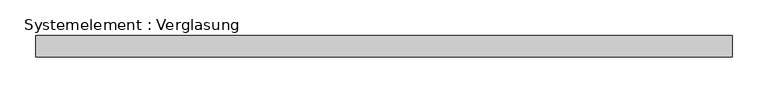
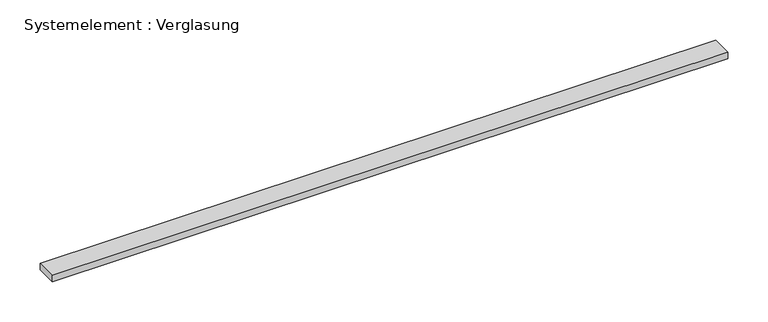
"""IFC4 building model written with IfcOpenShell, lengths in millimetres: plate geometry, Systemelement : Verglasung."""

from ifc_helpers import new_model, si_unit, origin, origin_with_axes, place, context, project, spatial, polyline, outline, extrude, source, transform, mapped, element, save


def systemelement_verglasung_579ed9d4(model_context):
    return source(origin(), model_context, "Body", "SweptSolid", [
        extrude(outline(polyline([(486.6118989, -15.0), (-486.6118989, -15.0), (-486.6118989, 15.0), (486.6118989, 15.0), (486.6118989, -15.0)])), origin_with_axes(), (0.0, 0.0, 1.0), 10.0),
    ])


if __name__ == "__main__":
    model = new_model("IFC4")
    model_context = context("Model", 3, world=origin())
    ifc_project = project(units=[si_unit("LENGTHUNIT", "METRE", prefix="MILLI")], contexts=[model_context])
    site = spatial("IfcSite", under=ifc_project)
    building = spatial("IfcBuilding", under=site)
    placement = place(None, origin())
    systemelement_verglasung_shape = systemelement_verglasung_579ed9d4(model_context)
    element("IfcPlate", 1, ObjectType="Systemelement : Verglasung", at=placement, inside=building, context=model_context, shape_type="MappedRepresentation", body=[
        mapped(systemelement_verglasung_shape, transform((0.0, 0.0, 0.0), x_axis=(1.0, 0.0, 0.0), y_axis=(0.0, 1.0, 0.0), z_axis=(0.0, 0.0, 1.0))),
    ])
    save(model, "model.ifc")

# Revit data of these elements
# Type "Systemelement : Verglasung"
#   Construction Type Id = "GSP4R"
#   Analytic Construction = "1/8 Zoll Pilkington-Verglasung einfach"
#   Visual Light Transmittance = 0.9
#   Solar Heat Gain Coefficient = 0.86
#   Heat Transfer Coefficient (U) = 6.7069 W/(m²·K)
# Element 1 (IfcPlate, "Systemelement : Verglasung")
#   Materials on its faces: "Glas"
# Materials
#   "Glas": class "Glas", colour RGB 0 0 255, transparency 0.75, Comments = "Render-Darstellung nicht aktualisiert ", Cost = 0
